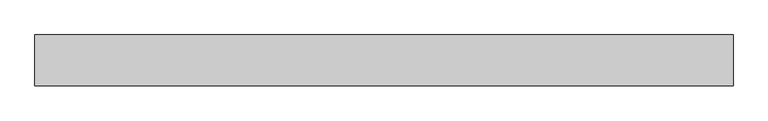
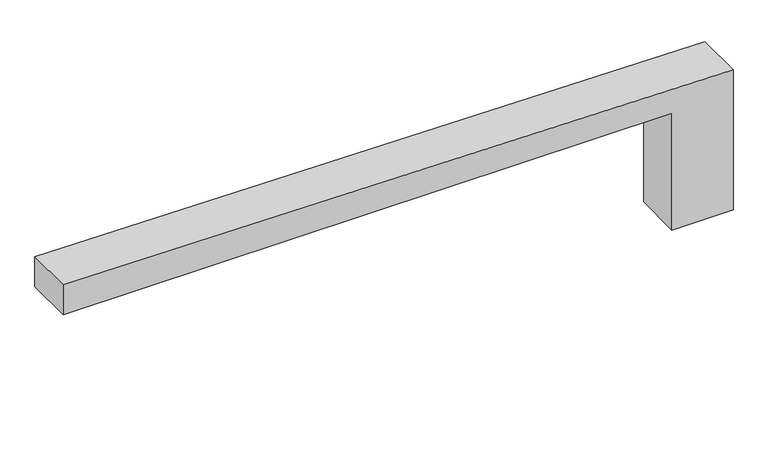
"""IFC4 building model written with IfcOpenShell, lengths in millimetres: proxy geometry, Generic Models 311:Generic Models 311:155231 : Generic Models 311:Generic Models 311:155231."""

from ifc_helpers import new_model, si_unit, frame, origin, place, context, project, spatial, polyline, outline, extrude, source, transform, mapped, element, save


def generic_models_1d2b1236(model_context):
    return source(origin(), model_context, "Body", "SweptSolid", [
        extrude(outline(polyline([(457.4693939, 8531.1032131), (501.65, 4365.503213), (304.8, 4365.503213), (304.8, 8150.1032131), (-463.1887049, 8150.1032131), (-463.1887049, 8531.1032131), (457.4693939, 8531.1032131)])), frame((0.0, -3919.5173293, 0.0), z_axis=(0.0, 1.0, 0.0), x_axis=(0.0, 0.0, 1.0)), (0.0, 0.0, 1.0), 304.8),
    ])


if __name__ == "__main__":
    model = new_model("IFC4")
    model_context = context("Model", 3, world=origin())
    ifc_project = project(units=[si_unit("LENGTHUNIT", "METRE", prefix="MILLI")], contexts=[model_context])
    site = spatial("IfcSite", under=ifc_project)
    building = spatial("IfcBuilding", under=site)
    placement = place(None, origin())
    generic_models_shape = generic_models_1d2b1236(model_context)
    element("IfcBuildingElementProxy", 1, Name="Generic Models 311:Generic Models 311:155231 : Generic Models 311:Generic Models 311:155231", ObjectType="Generic Models 311:Generic Models 311:155231 : Generic Models 311:Generic Models 311:155231", at=placement, inside=building, context=model_context, shape_type="MappedRepresentation", body=[
        mapped(generic_models_shape, transform((0.0, 0.0, 0.0), x_axis=(1.0, 0.0, 0.0), y_axis=(0.0, 1.0, 0.0), z_axis=(0.0, 0.0, 1.0))),
    ])
    save(model, "model.ifc")

# Revit data of these elements
# Type "Generic Models 311:Generic Models 311:155231 : Generic Models 311:Generic Models 311:155231"
#   NameOverride = "Generic Models 311:Generic Models 311:155231"
#   ObjectTypeOverride = "Generic Models 311:Generic Models 311"
#   Reference = "Generic Models 311"
#   Category = "Generic Models"
#   Tag = "155231"
# Element 1 (IfcBuildingElementProxy, "Generic Models 311:Generic Models 311:155231 : Generic Models 311:Generic Models 311:155231")
#   Materials on its faces: "_CONCRETE SLAB W/ WIRE MESH (SEE STRUCT. DWGS) - SLOPE 1% AWAY FROM BUILDING 9884"
# Materials
#   "_CONCRETE SLAB W/ WIRE MESH (SEE STRUCT. DWGS) - SLOPE 1% AWAY FROM BUILDING 9884": class "Unassigned", colour RGB 191 191 191, transparency 0
